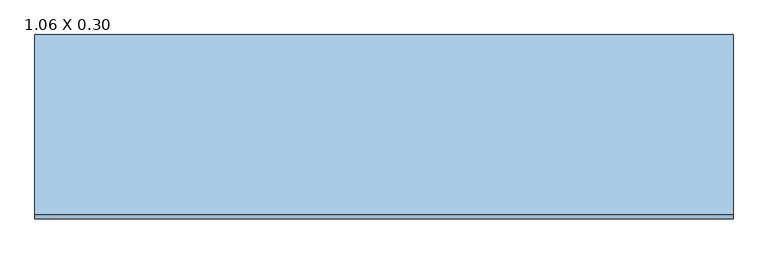
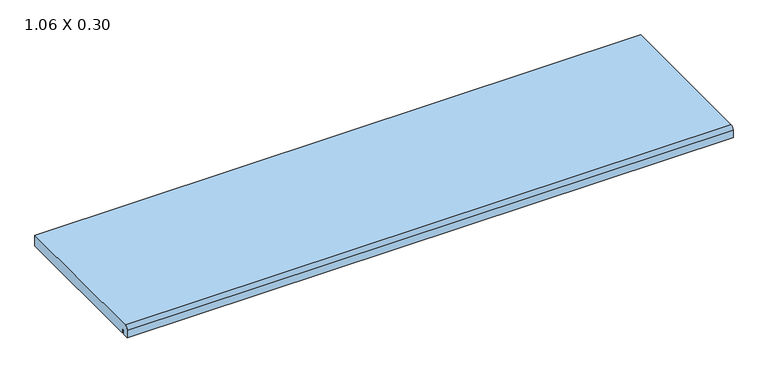
"""IFC4 building model written with IfcOpenShell, lengths in millimetres: window geometry, .CC_ND 300_PEDRA_PEITORIL RETO : 1.06 X 0.30."""

from ifc_helpers import new_model, si_unit, point, frame, frame_2d, origin, place, context, project, spatial, polyline, circle_curve, trimmed, segment, composite_curve, outline, extrude, source, transform, mapped, element, save


def window_1_06_x_0_30_7e01d648(model_context):
    return source(origin(), model_context, "Body", "SweptSolid", [
        extrude(outline(composite_curve([segment(polyline([(-132.5083081, 1480.0), (-132.5083081, 1488.1993124), (-137.2619526, 1488.1993124), (-137.2619526, 1480.0), (-148.0, 1480.0), (-148.0, 1493.3808343)]), True, "CONTINUOUS"), segment(trimmed(circle_curve(frame_2d((-141.3808343, 1493.3808343)), 6.6191657), [point((-148.0, 1493.3808343))], [point((-141.3808343, 1500.0))], False, "CARTESIAN"), True, "CONTINUOUS"), segment(polyline([(-141.3808343, 1500.0), (132.0, 1500.0), (132.0, 1480.0), (-132.5083081, 1480.0)]), True, "CONTINUOUS")], self_intersect=False)), frame((-530.0, 0.0, 0.0), z_axis=(1.0, 0.0, 0.0), x_axis=(0.0, 1.0, 0.0)), (0.0, 0.0, 1.0), 1060.0),
    ])


if __name__ == "__main__":
    model = new_model("IFC4")
    model_context = context("Model", 3, world=origin())
    ifc_project = project(units=[si_unit("LENGTHUNIT", "METRE", prefix="MILLI")], contexts=[model_context])
    site = spatial("IfcSite", under=ifc_project)
    building = spatial("IfcBuilding", under=site)
    placement = place(None, origin())
    window_1_06_x_0_30_shape = window_1_06_x_0_30_7e01d648(model_context)
    element("IfcWindow", 1, ObjectType=".CC_ND 300_PEDRA_PEITORIL RETO : 1.06 X 0.30", at=placement, inside=building, context=model_context, shape_type="MappedRepresentation", body=[
        mapped(window_1_06_x_0_30_shape, transform((0.0, 0.0, 0.0), x_axis=(1.0, 0.0, 0.0), y_axis=(0.0, 1.0, 0.0), z_axis=(0.0, 0.0, 1.0))),
    ])
    save(model, "model.ifc")

# Revit data of these elements
# Type ".CC_ND 300_PEDRA_PEITORIL RETO : 1.06 X 0.30"
#   Type Mark = "68"
#   Largura da pedra [instance default] = 0.26 m
#   Extensão interior peitoril [instance default] = 0.03 m
#   Extensão exterior peitoril [instance default] = 0.03 m
#   Espessura = 0.02 m
#   Comprimento = 1.06 m
#   Altura-padrão do peitoril = 1.48 m
#   Peitoril = .GRANITO_BRANCO_ITAUNAS
#   Rough Width = 0
#   Rough Height = 0
#   Height = 0
#   Wall Closure = (empty or 0)
#   Width = 0
# Element 1 (IfcWindow, ".CC_ND 300_PEDRA_PEITORIL RETO : 1.06 X 0.30")
#   Largura da pedra = 0.28 m
#   Extensão interior peitoril = 0.014 m
#   Materials on its faces: ".GRANITO_BRANCO_ITAUNAS"
# Materials
#   ".GRANITO_BRANCO_ITAUNAS": class ".CC_PEDRA REVEST.", colour RGB 202 195 174, transparency 0, Description = "Revestimento em granito", Cost = 0
